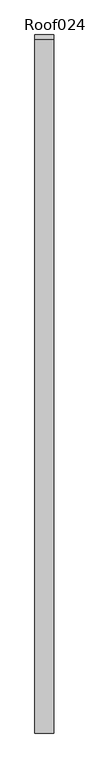
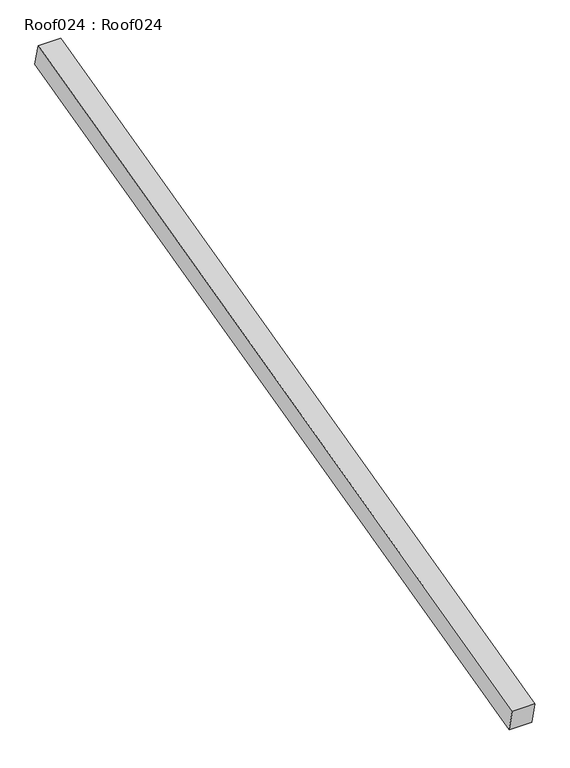
"""IFC4 building model written with IfcOpenShell, lengths in millimetres: proxy geometry, Roof024 : Roof024."""

from ifc_helpers import new_model, si_unit, frame, origin, place, context, project, spatial, polyline, outline, extrude, source, transform, mapped, element, save


def roof024_roof024_101e4ed5(model_context):
    return source(origin(), model_context, "Body", "SweptSolid", [
        extrude(outline(polyline([(-5247.7454625, 42918.7637785), (-3387.8525218, 43383.7351117), (-3374.6403653, 43330.8858071), (-5234.533306, 42865.9144738), (-5247.7454625, 42918.7637785)])), frame((13580.6064453, 0.0, 0.0), z_axis=(1.0, 0.0, 0.0), x_axis=(0.0, 1.0, 0.0)), (0.0, 0.0, 1.0), 50.8),
    ])


if __name__ == "__main__":
    model = new_model("IFC4")
    model_context = context("Model", 3, world=origin())
    ifc_project = project(units=[si_unit("LENGTHUNIT", "METRE", prefix="MILLI")], contexts=[model_context])
    site = spatial("IfcSite", under=ifc_project)
    building = spatial("IfcBuilding", under=site)
    placement = place(None, origin())
    roof024_roof024_shape = roof024_roof024_101e4ed5(model_context)
    element("IfcBuildingElementProxy", 1, Name="Roof024 : Roof024", ObjectType="Roof024 : Roof024", at=placement, inside=building, context=model_context, shape_type="MappedRepresentation", body=[
        mapped(roof024_roof024_shape, transform((0.0, 0.0, 0.0), x_axis=(1.0, 0.0, 0.0), y_axis=(0.0, 1.0, 0.0), z_axis=(0.0, 0.0, 1.0))),
    ])
    save(model, "model.ifc")

# Revit data of these elements
# Type "Roof024 : Roof024"
#   NameOverride = "Roof024"
# Element 1 (IfcBuildingElementProxy, "Roof024 : Roof024")
#   Materials on its faces: "STANDING SEAM METAL ROOF"
# Materials
#   "STANDING SEAM METAL ROOF": class "Unassigned", colour RGB 128 128 128, transparency 0
